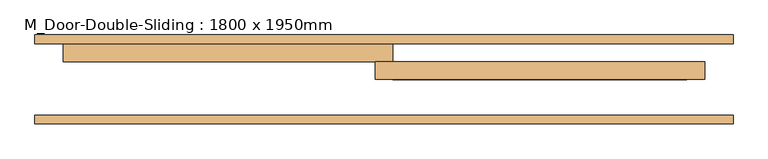
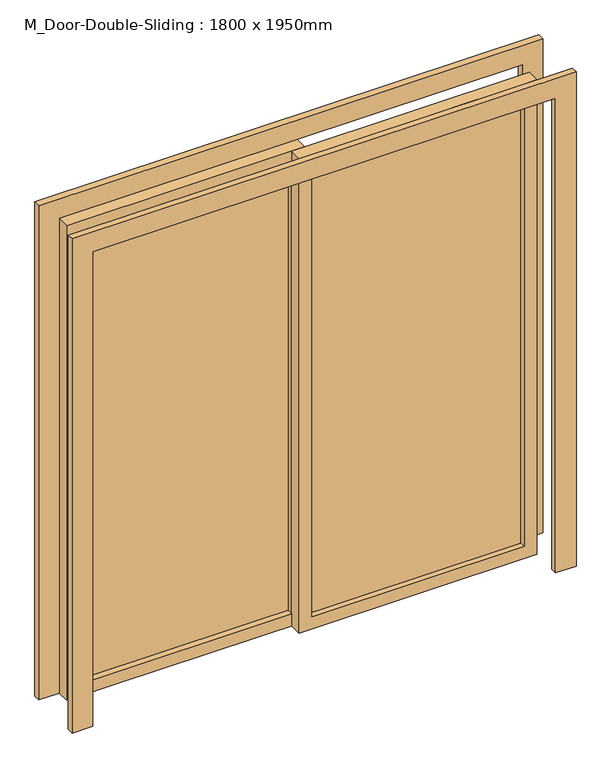
"""IFC4 building model written with IfcOpenShell, lengths in millimetres: door geometry, M_Door-Double-Sliding : 1800 x 1950mm."""

from ifc_helpers import new_model, si_unit, frame, origin, place, context, project, spatial, polyline, outline, extrude, source, transform, mapped, element, save


def m_door_double_sliding_1800_x_1950mm_ddb0fbbc(model_context):
    return source(origin(), model_context, "Body", "SweptSolid", [
        extrude(outline(polyline([(0.0, -980.0), (0.0, -900.0), (1950.0, -900.0), (1950.0, 900.0), (0.0, 900.0), (0.0, 980.0), (2030.0, 980.0), (2030.0, -980.0), (0.0, -980.0)])), frame((0.0, 2.0, 0.0), z_axis=(0.0, 1.0, 0.0), x_axis=(0.0, 0.0, 1.0)), (0.0, 0.0, 1.0), 25.0),
        extrude(outline(polyline([(0.0, 980.0), (2030.0, 980.0), (2030.0, -980.0), (0.0, -980.0), (0.0, -900.0), (1950.0, -900.0), (1950.0, 900.0), (0.0, 900.0), (0.0, 980.0)])), frame((0.0, 227.0, 0.0), z_axis=(0.0, 1.0, 0.0), x_axis=(0.0, 0.0, 1.0)), (0.0, 0.0, 1.0), 25.0),
        extrude(outline(polyline([(1950.0, -25.0), (0.0, -25.0), (0.0, 900.0), (1950.0, 900.0), (1950.0, -25.0)]), holes=[polyline([(1900.0, 25.0), (1900.0, 850.0), (50.0, 850.0), (50.0, 25.0), (1900.0, 25.0)])]), frame((0.0, 127.0, 0.0), z_axis=(0.0, 1.0, 0.0), x_axis=(0.0, 0.0, 1.0)), (0.0, 0.0, 1.0), 50.0),
        extrude(outline(polyline([(1950.0, 25.0), (1950.0, -900.0), (0.0, -900.0), (0.0, 25.0), (1950.0, 25.0)]), holes=[polyline([(1900.0, -25.0), (50.0, -25.0), (50.0, -850.0), (1900.0, -850.0), (1900.0, -25.0)])]), frame((0.0, 177.0, 0.0), z_axis=(0.0, 1.0, 0.0), x_axis=(0.0, 0.0, 1.0)), (0.0, 0.0, 1.0), 50.0),
        extrude(outline(polyline([(25.0, 155.175), (850.0, 155.175), (850.0, 148.825), (25.0, 148.825), (25.0, 155.175)])), frame((0.0, 0.0, 50.0), z_axis=(0.0, 0.0, 1.0), x_axis=(1.0, 0.0, 0.0)), (0.0, 0.0, 1.0), 1850.0),
        extrude(outline(polyline([(-25.0, 200.025), (-850.0, 200.025), (-850.0, 206.375), (-25.0, 206.375), (-25.0, 200.025)])), frame((0.0, 0.0, 50.0), z_axis=(0.0, 0.0, 1.0), x_axis=(1.0, 0.0, 0.0)), (0.0, 0.0, 1.0), 1850.0),
    ])


if __name__ == "__main__":
    model = new_model("IFC4")
    model_context = context("Model", 3, world=origin())
    ifc_project = project(units=[si_unit("LENGTHUNIT", "METRE", prefix="MILLI")], contexts=[model_context])
    site = spatial("IfcSite", under=ifc_project)
    building = spatial("IfcBuilding", under=site)
    placement = place(None, origin())
    m_door_double_sliding_1800_x_1950mm_shape = m_door_double_sliding_1800_x_1950mm_ddb0fbbc(model_context)
    element("IfcDoor", 1, ObjectType="M_Door-Double-Sliding : 1800 x 1950mm", at=placement, inside=building, context=model_context, shape_type="MappedRepresentation", body=[
        mapped(m_door_double_sliding_1800_x_1950mm_shape, transform((0.0, 0.0, 0.0), x_axis=(1.0, 0.0, 0.0), y_axis=(0.0, 1.0, 0.0), z_axis=(0.0, 0.0, 1.0))),
    ])
    save(model, "model.ifc")

# Revit data of these elements
# Type "M_Door-Double-Sliding : 1800 x 1950mm"
#   Type Mark = "42"
#   Construction Type Id = "opn-d45"
#   Assembly Code = "C1020"
#   Analytic Construction = "Wood frame, double glass door "
#   Thickness = 50 mm
#   Thermal Resistance (R) = 0.31964 (m²·K)/W
#   Heat Transfer Coefficient (U) = 3.12872 W/(m²·K)
#   Height = 1950 mm
#   Rail Width = 50 mm
#   Stiles = 50 mm
#   Trim Projection Ext = 25 mm
#   Trim Projection Int = 25 mm
#   Trim Width = 80 mm
#   Width = 1800 mm
#   Glazing = Glass
#   Panel Material = Wood - Birch - Solid Stained Light Low Gloss
#   Trim Material = Paint - Sienna
#   Visual Light Transmittance = 0
#   Solar Heat Gain Coefficient = 0
#   Function = (empty or 0)
#   Wall Closure = (empty or 0)
# Element 1 (IfcDoor, "M_Door-Double-Sliding : 1800 x 1950mm")
#   Materials on its faces: "Paint - Sienna", "Wood - Birch - Solid Stained Light Low Gloss", "Glass"
# Materials
#   "Glass": class "Glass", colour RGB 55 55 255, transparency 0.9, Description = "Soda Lime Glass", Cost = 0
#   "Wood - Birch - Solid Stained Light Low Gloss": class "Wood", colour RGB 210 159 95, transparency 0, Cost = 0
#   "Paint - Sienna": class "Miscellaneous", colour RGB 118 70 51, transparency 0, Cost = 0
